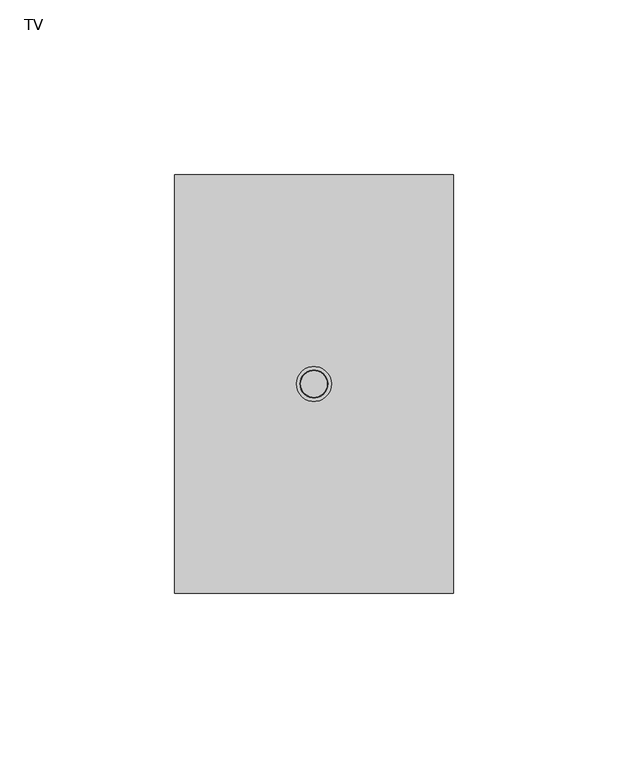
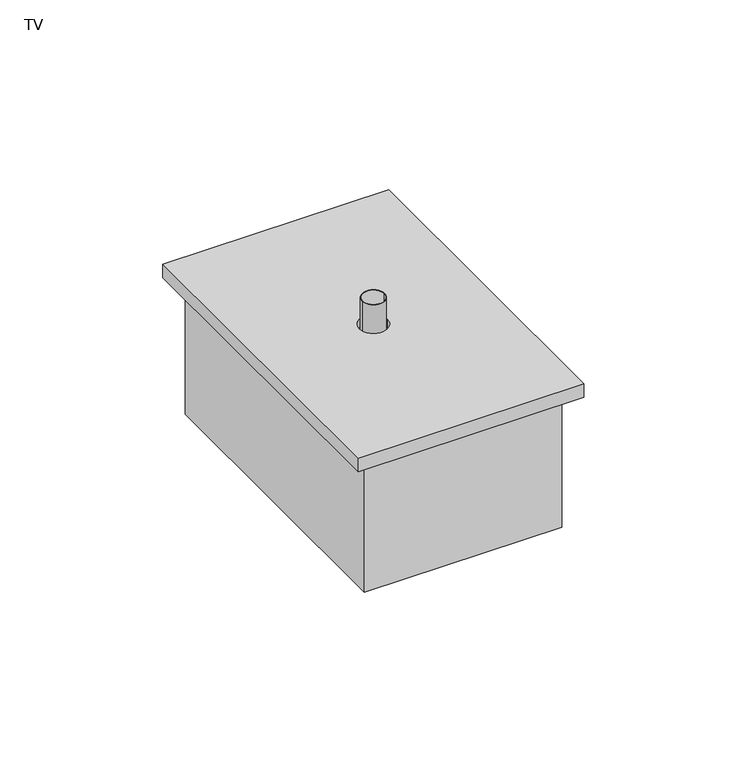
"""IFC4 building model written with IfcOpenShell, lengths in millimetres: proxy geometry, CAIXA VERTICE V7 : TV."""

from ifc_helpers import new_model, si_unit, point, frame, frame_2d, origin, origin_with_axes, place, context, project, spatial, polyline, circle_curve, trimmed, segment, composite_curve, outline, extrude, faceted_brep, source, transform, mapped, element, save
from ifc_brep_helpers import plane_surface, revolved_surface, advanced_brep


def tv_5bebb12c(model_context):
    return source(origin(), model_context, "Body", "SolidModel", [
        extrude(outline(composite_curve([segment(trimmed(circle_curve(frame_2d((0.0, -1100.0)), 4.0), [point((-4.0, -1100.0))], [point((4.0, -1100.0))], False, "CARTESIAN"), True, "CONTINUOUS"), segment(trimmed(circle_curve(frame_2d((0.0, -1100.0)), 4.0), [point((4.0, -1100.0))], [point((-4.0, -1100.0))], False, "CARTESIAN"), True, "CONTINUOUS")], self_intersect=False), holes=[composite_curve([segment(trimmed(circle_curve(frame_2d((0.0, -1100.0)), 3.8), [point((-3.8, -1100.0))], [point((3.8, -1100.0))], True, "CARTESIAN"), True, "CONTINUOUS"), segment(trimmed(circle_curve(frame_2d((0.0, -1100.0)), 3.8), [point((3.8, -1100.0))], [point((-3.8, -1100.0))], True, "CARTESIAN"), True, "CONTINUOUS")], self_intersect=False)]), origin_with_axes(), (0.0, 0.0, 1.0), 15.0),
        faceted_brep([(33.0, -1047.0, -48.0), (-33.0, -1047.0, -48.0), (-33.0, -1153.0, -48.0), (33.0, -1153.0, -48.0), (35.0, -1155.0, -50.0), (-35.0, -1155.0, -50.0), (-35.0, -1045.0, -50.0), (35.0, -1045.0, -50.0), (35.0, -1155.0, 0.0), (-35.0, -1155.0, 0.0), (-35.0, -1045.0, 0.0), (35.0, -1045.0, 0.0), (33.0, -1153.0, 0.0), (-33.0, -1153.0, 0.0), (-33.0, -1047.0, 0.0), (33.0, -1047.0, 0.0)], [[[0, 1, 2, 3]], [[4, 5, 6, 7]], [[4, 8, 9, 5]], [[9, 10, 6, 5]], [[10, 11, 7, 6]], [[11, 8, 4, 7]], [[8, 11, 10, 9], [12, 13, 14, 15]], [[15, 0, 3, 12]], [[14, 1, 0, 15]], [[13, 2, 1, 14]], [[12, 3, 2, 13]]]),
        advanced_brep(
        [(40.0, -1160.0, 5.0), (40.0, -1040.0, 5.0), (-40.0, -1040.0, 5.0), (-40.0, -1160.0, 5.0), (5.0, -1100.0, 5.0), (-5.0, -1100.0, 5.0), (-40.0, -1160.0, 0.0), (-40.0, -1040.0, 0.0), (40.0, -1040.0, 0.0), (40.0, -1160.0, 0.0), (5.0, -1100.0, 2.0), (-5.0, -1100.0, 2.0)],
        [
            (0, 1),
            (1, 2),
            (2, 3),
            (3, 0),
            (4, 5, circle_curve(frame((0.0, -1100.0, 5.0), z_axis=(0.0, 0.0, -1.0), x_axis=(1.0, 0.0, 0.0)), 5.0)),
            (5, 4, circle_curve(frame((0.0, -1100.0, 5.0), z_axis=(0.0, 0.0, -1.0), x_axis=(1.0, 0.0, 0.0)), 5.0)),
            (6, 7),
            (7, 8),
            (8, 9),
            (9, 6),
            (3, 6),
            (9, 0),
            (2, 7),
            (1, 8),
            (10, 4),
            (5, 11),
            (11, 10, circle_curve(frame((0.0, -1100.0, 2.0), z_axis=(0.0, 0.0, -1.0), x_axis=(1.0, 0.0, 0.0)), 5.0)),
            (11, 10, circle_curve(frame((0.0, -1100.0, 2.0), z_axis=(0.0, 0.0, 1.0), x_axis=(1.0, 0.0, 0.0)), 5.0)),
        ],
        [
            plane_surface(frame((-60.0, -1160.0, 5.0), z_axis=(0.0, 0.0, 1.0), x_axis=(-1.0, 0.0, 0.0))),
            plane_surface(frame((-60.0, -1160.0, 0.0), z_axis=(0.0, 0.0, -1.0), x_axis=(1.0, 0.0, 0.0))),
            plane_surface(frame((40.0, -1160.0, 5.0), z_axis=(0.0, -1.0, 0.0), x_axis=(0.0, 0.0, -1.0))),
            plane_surface(frame((-40.0, -1160.0, 5.0), z_axis=(-1.0, 0.0, 0.0), x_axis=(0.0, 0.0, -1.0))),
            plane_surface(frame((-40.0, -1040.0, 5.0), z_axis=(0.0, 1.0, 0.0), x_axis=(0.0, 0.0, -1.0))),
            plane_surface(frame((40.0, -1040.0, 5.0), z_axis=(1.0, 0.0, 0.0), x_axis=(0.0, 0.0, -1.0))),
            revolved_surface(polyline([(5.0, -1100.0, 5.0), (5.0, -1100.0, 2.0)]), (0.0, -1100.0, 2.0), (0.0, 0.0, 1.0)),
            plane_surface(frame((5.0, -1100.0, 2.0), z_axis=(0.0, 0.0, 1.0), x_axis=(0.0, 1.0, 0.0))),
        ],
        [
            (0, [[1, 2, 3, 4], [5, 6]]),
            (1, [[7, 8, 9, 10]]),
            (2, [[11, -10, 12, -4]]),
            (3, [[13, -7, -11, -3]]),
            (4, [[14, -8, -13, -2]]),
            (5, [[-12, -9, -14, -1]]),
            (6, [[15, -6, 16, 17]]),
            (7, [[18, -17]]),
            (6, [[-16, -5, -15, -18]]),
        ],
    ),
    ])


if __name__ == "__main__":
    model = new_model("IFC4")
    model_context = context("Model", 3, world=origin())
    ifc_project = project(units=[si_unit("LENGTHUNIT", "METRE", prefix="MILLI")], contexts=[model_context])
    site = spatial("IfcSite", under=ifc_project)
    building = spatial("IfcBuilding", under=site)
    placement = place(None, origin())
    tv_shape = tv_5bebb12c(model_context)
    element("IfcBuildingElementProxy", 1, Name="CAIXA VERTICE V7 : TV", ObjectType="CAIXA VERTICE V7 : TV", at=placement, inside=building, context=model_context, shape_type="MappedRepresentation", body=[
        mapped(tv_shape, transform((0.0, 0.0, 0.0), x_axis=(1.0, 0.0, 0.0), y_axis=(0.0, 1.0, 0.0), z_axis=(0.0, 0.0, 1.0))),
    ])
    save(model, "model.ifc")

# Revit data of these elements
# Type "CAIXA VERTICE V7 : TV"
#   URL = "www.facebook.com/verticetreinamentos"
#   SEÇÃO [instance default] = ""
#   Rotação [instance default] = 0.00°
#   LARGURA DA TAMPA = 0.08 m
#   BORDA = 0.01 m
#   ALTURA DE INSTALAÇÃO [instance default] = 1.10 m
#   Distância Anotação [instance default] = 0.0015 m
#   ALTURA DA TAMPA = 0.12 m
#   Vertical [instance default] = yes
#   VER SEÇÃO [instance default] = no
#   SHADE ESQ [instance default] = no
#   SHADE DIR [instance default] = yes
#   HORIZONTAL [instance default] = no
#   ANDAR COM A LEGENDA [instance default] = 0
#   Material Tampa [instance default] = Plástico, branco opaco
#   Caixa = element 1798535
#   Anotação = element 1798534
#   Default Elevation = 0
# Element 1 (IfcBuildingElementProxy, "CAIXA VERTICE V7 : TV")
#   Materials on its faces: "Plástico, branco opaco"
# Materials
#   "Plástico, branco opaco": class "Plástico", colour RGB 120 120 120, transparency 0, Description = "Plastic, generic, opaque white", Cost = 0
